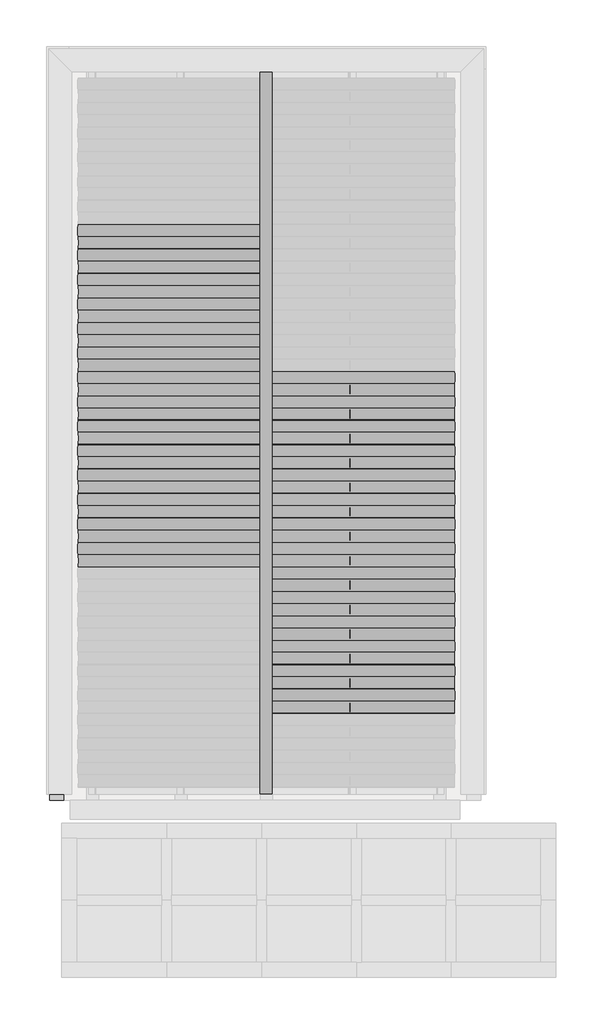
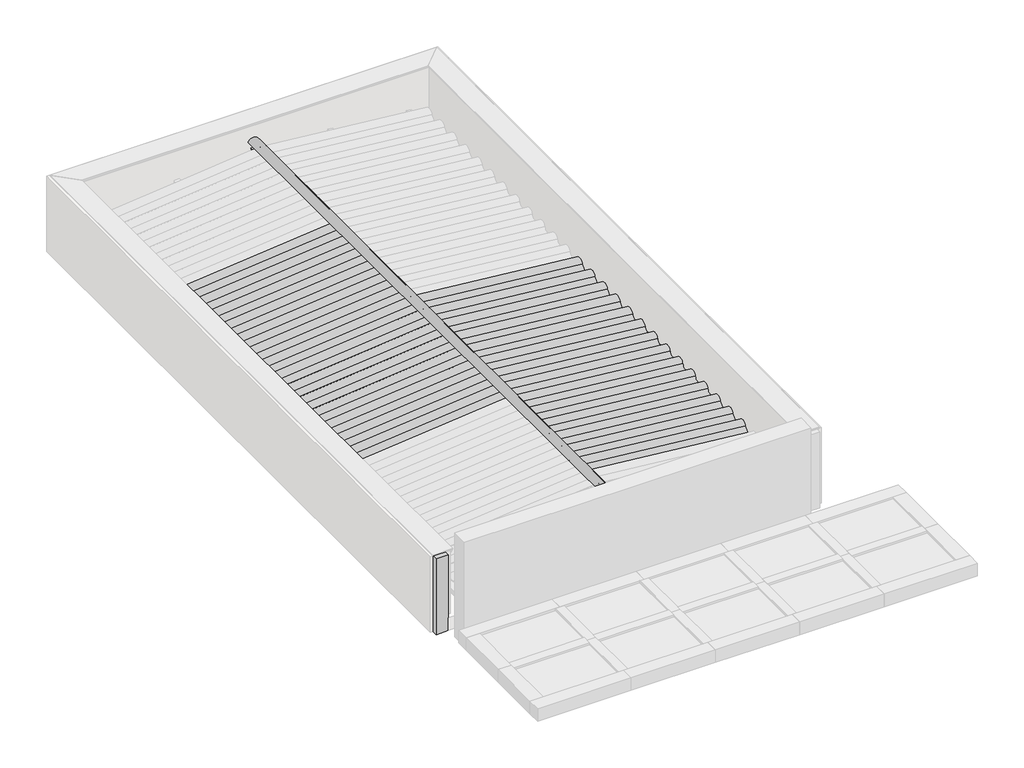
# One storey, part 2 of 3: 37 beams, 7 columns.
"""IFC4 building model written with IfcOpenShell, lengths in millimetres."""

import ifcopenshell
import ifcopenshell.guid

model = None  # the IFC model being written
_history = None  # IfcOwnerHistory: only IFC2X3 demands one
_inside = {}  # id of a spatial element -> (the spatial element, [elements in it])
_under = {}  # id of a project, library or spatial element -> (it, [spatial elements below it])
_declared = {}  # id of a project -> (the project, [libraries it declares])
_typed = {}  # id of a type object -> (the type object, [elements of that type])
_made_of = {}  # id of a material, layer set ... -> (it, [elements and type objects made of it])


def new_model(schema):
    """Start an empty IFC model of exactly this schema.

    Asked for "IFC4X3", IfcOpenShell would pick the latest addendum, in which some entities
    have other attributes; the version numbers below select the first issue.
    IFC2X3 requires an IfcOwnerHistory on every rooted entity: one is made here for all.
    """
    global model, _history
    if schema == "IFC4X3":
        model = ifcopenshell.file(schema_version=(4, 3, 0, 0))
    else:
        model = ifcopenshell.file(schema=schema)
    _inside.clear()
    _under.clear()
    _declared.clear()
    _typed.clear()
    _made_of.clear()
    _history = None
    if model.schema == "IFC2X3":
        org = make("IfcOrganization", Name="unknown")
        user = make(
            "IfcPersonAndOrganization",
            ThePerson=make("IfcPerson", FamilyName="unknown"),
            TheOrganization=org,
        )
        app = make(
            "IfcApplication",
            ApplicationDeveloper=org,
            Version="unknown",
            ApplicationFullName="unknown",
            ApplicationIdentifier="unknown",
        )
        _history = make(
            "IfcOwnerHistory",
            OwningUser=user,
            OwningApplication=app,
            ChangeAction="ADDED",
            CreationDate=0,
        )
    return model


def make(cls, **values):
    """One entity of the class cls with the attributes given. An attribute that is None is left unset."""
    return model.create_entity(
        cls, **{name: value for name, value in values.items() if value is not None}
    )


def rooted(cls, **values):
    """An entity with a GlobalId (a new one), such as an element, a storey or a relation."""
    return make(cls, GlobalId=ifcopenshell.guid.new(), OwnerHistory=_history, **values)


def si_unit(unit_type, name, prefix=None):
    """IfcSIUnit, for example si_unit("LENGTHUNIT", "METRE", prefix="MILLI")."""
    return make("IfcSIUnit", UnitType=unit_type, Prefix=prefix, Name=name)


def assignment(units):
    """IfcUnitAssignment: the units of a project."""
    return None if units is None else make("IfcUnitAssignment", Units=units)


def point(xyz):
    """IfcCartesianPoint."""
    return None if xyz is None else make("IfcCartesianPoint", Coordinates=xyz)


def direction(xyz):
    """IfcDirection."""
    return None if xyz is None else make("IfcDirection", DirectionRatios=xyz)


def frame(location, z_axis=None, x_axis=None):
    """IfcAxis2Placement3D, a coordinate frame: its origin and axes. An axis left out is left unset."""
    return make(
        "IfcAxis2Placement3D",
        Location=point(location),
        Axis=direction(z_axis),
        RefDirection=direction(x_axis),
    )


def frame_2d(location, x_axis=None):
    """IfcAxis2Placement2D, a coordinate frame in the plane: its origin and x axis."""
    return make(
        "IfcAxis2Placement2D", Location=point(location), RefDirection=direction(x_axis)
    )


def origin():
    """The frame at (0, 0, 0) with its axes left unset."""
    return frame((0.0, 0.0, 0.0))


def place(relative_to, where):
    """IfcLocalPlacement: puts the frame where relative to a parent placement (None: the world)."""
    return make(
        "IfcLocalPlacement", PlacementRelTo=relative_to, RelativePlacement=where
    )


def context(
    kind, dimensions, precision=None, world=None, true_north=None, identifier=None
):
    """IfcGeometricRepresentationContext, for example the 3D "Model" context."""
    return make(
        "IfcGeometricRepresentationContext",
        ContextIdentifier=identifier,
        ContextType=kind,
        CoordinateSpaceDimension=dimensions,
        Precision=precision,
        WorldCoordinateSystem=world,
        TrueNorth=true_north,
    )


def project(units=None, contexts=None):
    """IfcProject with its units and contexts."""
    return rooted(
        "IfcProject",
        Name="project",
        RepresentationContexts=contexts,
        UnitsInContext=assignment(units),
    )


def spatial(cls, under=None, at=None, **own):
    """A site, building, storey or space (cls), placed at a placement, below another one or the project."""
    s = rooted(cls, ObjectPlacement=at, **own)
    if under is not None:
        _under.setdefault(under.id(), (under, []))[1].append(s)
    return s


def polyline(points):
    """IfcPolyline through the points."""
    return make("IfcPolyline", Points=[point(p) for p in points])


def circle_curve(where, radius):
    """IfcCircle in the frame where."""
    return make("IfcCircle", Position=where, Radius=radius)


def trimmed(basis, trim1, trim2, sense, master):
    """IfcTrimmedCurve: the piece of a basis curve between two trims."""
    return make(
        "IfcTrimmedCurve",
        BasisCurve=basis,
        Trim1=trim1,
        Trim2=trim2,
        SenseAgreement=sense,
        MasterRepresentation=master,
    )


def segment(curve, same_sense, transition):
    """IfcCompositeCurveSegment."""
    return make(
        "IfcCompositeCurveSegment",
        Transition=transition,
        SameSense=same_sense,
        ParentCurve=curve,
    )


def composite_curve(segments, self_intersect=None):
    """IfcCompositeCurve: segments joined end to end."""
    return make("IfcCompositeCurve", Segments=segments, SelfIntersect=self_intersect)


def outline(outer, holes=None, kind="AREA"):
    """IfcArbitraryClosedProfileDef: a profile drawn as a closed curve; with holes, ...WithVoids."""
    if holes is None:
        return make("IfcArbitraryClosedProfileDef", ProfileType=kind, OuterCurve=outer)
    return make(
        "IfcArbitraryProfileDefWithVoids",
        ProfileType=kind,
        OuterCurve=outer,
        InnerCurves=holes,
    )


def extrude(swept, where, along, depth):
    """IfcExtrudedAreaSolid: the profile swept, set in the frame where, extruded along a direction by depth."""
    return make(
        "IfcExtrudedAreaSolid",
        SweptArea=swept,
        Position=where,
        ExtrudedDirection=direction(along),
        Depth=depth,
    )


def faces_of(points, faces, orient=None, outer=None):
    """IfcFace entities. A face is a list of loops; a loop is a list of indices into points, from 0.

    orient and outer hold one flag for each loop. By default every Orientation is true, the
    first loop of a face is its IfcFaceOuterBound and the others are IfcFaceBound.
    """
    made = []
    for i, loops in enumerate(faces):
        bounds = []
        for j, loop in enumerate(loops):
            is_outer = j == 0 if outer is None else outer[i][j]
            bounds.append(
                make(
                    "IfcFaceOuterBound" if is_outer else "IfcFaceBound",
                    Bound=make("IfcPolyLoop", Polygon=[points[k] for k in loop]),
                    Orientation=True if orient is None else orient[i][j],
                )
            )
        made.append(make("IfcFace", Bounds=bounds))
    return made


def faceted_brep(points, faces, orient=None, outer=None, voids=None):
    """IfcFacetedBrep: a solid bounded by flat faces; with voids (closed shells), ...WithVoids."""
    shared = [point(p) for p in points]
    hull = make("IfcClosedShell", CfsFaces=faces_of(shared, faces, orient, outer))
    if voids is None:
        return make("IfcFacetedBrep", Outer=hull)
    return make(
        "IfcFacetedBrepWithVoids",
        Outer=hull,
        Voids=[
            make(cls, CfsFaces=faces_of(shared, fs, o, b)) for cls, fs, o, b in voids
        ],
    )


def shape(context_of_items, identifier, shape_type, items):
    """IfcShapeRepresentation: the items that make up one representation, for example the "Body"."""
    return make(
        "IfcShapeRepresentation",
        ContextOfItems=context_of_items,
        RepresentationIdentifier=identifier,
        RepresentationType=shape_type,
        Items=items,
    )


def source(mapping_origin, context_of_items, identifier, shape_type, items):
    """IfcRepresentationMap: a shape defined once, which mapped items show again and again."""
    return make(
        "IfcRepresentationMap",
        MappingOrigin=mapping_origin,
        MappedRepresentation=shape(context_of_items, identifier, shape_type, items),
    )


def transform(
    local_origin,
    x_axis=None,
    y_axis=None,
    z_axis=None,
    scale=None,
    scale2=None,
    scale3=None,
    uniform=True,
):
    """IfcCartesianTransformationOperator3D, or its non-uniform kind. x_axis, y_axis, z_axis: its Axis1, 2, 3."""
    if uniform:
        return make(
            "IfcCartesianTransformationOperator3D",
            Axis1=direction(x_axis),
            Axis2=direction(y_axis),
            LocalOrigin=point(local_origin),
            Scale=scale,
            Axis3=direction(z_axis),
        )
    return make(
        "IfcCartesianTransformationOperator3DnonUniform",
        Axis1=direction(x_axis),
        Axis2=direction(y_axis),
        LocalOrigin=point(local_origin),
        Scale=scale,
        Axis3=direction(z_axis),
        Scale2=scale2,
        Scale3=scale3,
    )


def mapped(mapping_source, mapping_target):
    """IfcMappedItem: shows the shape of a source again, moved by a transform."""
    return make(
        "IfcMappedItem", MappingSource=mapping_source, MappingTarget=mapping_target
    )


def made_of(thing, what):
    """Note that an element or type object is made of a material, layer set ...; save() writes the relation."""
    if what is not None:
        _made_of.setdefault(what.id(), (what, []))[1].append(thing)
    return thing


def element(
    cls,
    number,
    at=None,
    inside=None,
    cuts=None,
    type_object=None,
    material=None,
    context=None,
    identifier="Body",
    shape_type=None,
    held_by="IfcProductDefinitionShape",
    body=None,
    shapes=None,
    **own,
):
    """One element of the class cls, such as IfcWall. Its Tag is "e" and its number.

    at: its placement. inside: the storey or other place that contains it. cuts: it is an
    opening in that element (IfcRelVoidsElement). A single representation is given by context,
    identifier, shape_type and body (its items); several are given by shapes. held_by: the class
    of the entity that holds the representations. save() writes the other relations.
    """
    e = rooted(cls, Tag="e%d" % number, ObjectPlacement=at, **own)
    if body is not None:
        shapes = [shape(context, identifier, shape_type, body)]
    if shapes is not None:
        e.Representation = make(held_by, Representations=shapes)
    if inside is not None:
        _inside.setdefault(inside.id(), (inside, []))[1].append(e)
    if cuts is not None:
        rooted(
            "IfcRelVoidsElement", RelatingBuildingElement=cuts, RelatedOpeningElement=e
        )
    if type_object is not None:
        _typed.setdefault(type_object.id(), (type_object, []))[1].append(e)
    return made_of(e, material)


def aggregate(whole, parts):
    """IfcRelAggregates: a whole, such as a stair, and the parts it consists of."""
    return rooted("IfcRelAggregates", RelatingObject=whole, RelatedObjects=parts)


def save(model, path):
    """Write the relations noted so far, then the file.

    IfcRelAggregates (storeys below a building ...), IfcRelContainedInSpatialStructure (elements
    in a storey), IfcRelDefinesByType, IfcRelAssociatesMaterial and IfcRelDeclares: one each for
    every whole, place, type object, material and project.
    """
    for whole, parts in _under.values():
        aggregate(whole, parts)
    for where, things in _inside.values():
        rooted(
            "IfcRelContainedInSpatialStructure",
            RelatedElements=things,
            RelatingStructure=where,
        )
    for kind, things in _typed.values():
        rooted("IfcRelDefinesByType", RelatedObjects=things, RelatingType=kind)
    for what, things in _made_of.values():
        rooted("IfcRelAssociatesMaterial", RelatedObjects=things, RelatingMaterial=what)
    for by, libraries in _declared.values():
        rooted("IfcRelDeclares", RelatingContext=by, RelatedDefinitions=libraries)
    model.write(path)


def cumeeira_telha_ondulada_fibrocimento_28917381(model_context):
    return source(origin(), model_context, "Body", "SweptSolid", [
        extrude(outline(composite_curve([segment(polyline([(58.3970135, 42.4437972), (53.9055884, 40.2467307)]), True, "CONTINUOUS"), segment(trimmed(circle_curve(frame_2d((-1.6029865, 13.0936483)), 61.7939461), [point((53.9055884, 40.2467307))], [point((-57.1115615, 40.2467307))], True, "CARTESIAN"), True, "CONTINUOUS"), segment(polyline([(-57.1115615, 40.2467307), (-61.6029865, 42.4437972)]), True, "CONTINUOUS"), segment(trimmed(circle_curve(frame_2d((-1.6029865, 13.0936483)), 66.7939461), [point((-61.6029865, 42.4437972))], [point((58.3970135, 42.4437972))], False, "CARTESIAN"), True, "CONTINUOUS")], self_intersect=False)), frame((-3626.5, 0.0, 0.0), z_axis=(1.0, 0.0, 0.0), x_axis=(0.0, 1.0, 0.0)), (0.0, 0.0, 1.0), 7253.0),
    ])


def viga_cumeeira_6x16cm_d80f05ee(model_context):
    return source(origin(), model_context, "Body", "SweptSolid", [
        extrude(outline(polyline([(3626.5, 30.0), (3626.5, -30.0), (-3626.5, -30.0), (-3626.5, 30.0), (3626.5, 30.0)])), frame((0.0, 0.0, -80.0), z_axis=(0.0, 0.0, 1.0), x_axis=(1.0, 0.0, 0.0)), (0.0, 0.0, 1.0), 160.0),
    ])


def column_1cffec27(model_context):
    return source(origin(), model_context, "Body", "SweptSolid", [
        extrude(outline(polyline([(30.0, 80.0), (30.0, -80.0), (-30.0, -80.0), (-30.0, 80.0), (30.0, 80.0)])), frame((0.0, 0.0, 3110.0), z_axis=(0.0, 0.0, 1.0), x_axis=(1.0, 0.0, 0.0)), (0.0, 0.0, 1.0), 238.0),
    ])


def column_35730ad5(model_context):
    return source(origin(), model_context, "Body", "SweptSolid", [
        extrude(outline(polyline([(30.0, 80.0), (30.0, -80.0), (-30.0, -80.0), (-30.0, 80.0), (30.0, 80.0)])), frame((0.0, 0.0, 3110.0), z_axis=(0.0, 0.0, 1.0), x_axis=(1.0, 0.0, 0.0)), (0.0, 0.0, 1.0), 197.9),
    ])


def column_00c463e4(model_context):
    return source(origin(), model_context, "Body", "SweptSolid", [
        extrude(outline(polyline([(30.0, 80.0), (30.0, -80.0), (-30.0, -80.0), (-30.0, 80.0), (30.0, 80.0)])), frame((0.0, 0.0, 3110.0), z_axis=(0.0, 0.0, 1.0), x_axis=(1.0, 0.0, 0.0)), (0.0, 0.0, 1.0), 109.8),
    ])


model = new_model("IFC4")

# Units and contexts
model_context = context("Model", 3, world=origin())
ifc_project = project(units=[si_unit("LENGTHUNIT", "METRE", prefix="MILLI")], contexts=[model_context])

# Site, building, storey
site = spatial("IfcSite", under=ifc_project)
building = spatial("IfcBuilding", under=site)
storey = spatial("IfcBuildingStorey", under=building, Name="COB. GARAGEM", Elevation=3050.0)

# Beams
placement = place(None, origin())
element("IfcBeam", 1, ObjectType="Madeira de lei : Berço 6x12cm", at=placement, inside=storey, context=model_context, shape_type="SweptSolid", body=[
    extrude(outline(polyline([(-9620.281307, 4423.9300153), (-9500.281307, 4423.9300153), (-9500.281307, 2423.9300153), (-9620.281307, 2423.9300153), (-9620.281307, 4423.9300153)])), frame((0.0, 0.0, 3050.0), z_axis=(0.0, 0.0, 1.0), x_axis=(1.0, 0.0, 0.0)), (0.0, 0.0, 1.0), 60.0),
])
element("IfcBeam", 2, ObjectType="Madeira de lei : Berço 6x12cm", at=placement, inside=storey, context=model_context, shape_type="SweptSolid", body=[
    extrude(outline(polyline([(-9620.281307, 2423.9300153), (-9500.281307, 2423.9300153), (-9500.281307, 423.9300153), (-9620.281307, 423.9300153), (-9620.281307, 2423.9300153)])), frame((0.0, 0.0, 3050.0), z_axis=(0.0, 0.0, 1.0), x_axis=(1.0, 0.0, 0.0)), (0.0, 0.0, 1.0), 60.0),
])
element("IfcBeam", 3, ObjectType="Madeira de lei : Berço 6x12cm", at=placement, inside=storey, context=model_context, shape_type="SweptSolid", body=[
    extrude(outline(polyline([(-8767.0824227, 4423.9300153), (-8647.0824227, 4423.9300153), (-8647.0824227, 2423.9300153), (-8767.0824227, 2423.9300153), (-8767.0824227, 4423.9300153)])), frame((0.0, 0.0, 3050.0), z_axis=(0.0, 0.0, 1.0), x_axis=(1.0, 0.0, 0.0)), (0.0, 0.0, 1.0), 60.0),
])
element("IfcBeam", 4, ObjectType="Madeira de lei : Berço 6x12cm", at=placement, inside=storey, context=model_context, shape_type="SweptSolid", body=[
    extrude(outline(polyline([(-10473.4801913, 4423.9300153), (-10353.4801913, 4423.9300153), (-10353.4801913, 2423.9300153), (-10473.4801913, 2423.9300153), (-10473.4801913, 4423.9300153)])), frame((0.0, 0.0, 3050.0), z_axis=(0.0, 0.0, 1.0), x_axis=(1.0, 0.0, 0.0)), (0.0, 0.0, 1.0), 60.0),
])
element("IfcBeam", 5, ObjectType="Madeira de lei : Berço 6x12cm", at=placement, inside=storey, context=model_context, shape_type="SweptSolid", body=[
    extrude(outline(polyline([(-11356.5301913, 4423.9300153), (-11236.5301913, 4423.9300153), (-11236.5301913, 2423.9300153), (-11356.5301913, 2423.9300153), (-11356.5301913, 4423.9300153)])), frame((0.0, 0.0, 3050.0), z_axis=(0.0, 0.0, 1.0), x_axis=(1.0, 0.0, 0.0)), (0.0, 0.0, 1.0), 60.0),
])
element("IfcBeam", 6, ObjectType="Madeira de lei : Berço 6x12cm", at=placement, inside=storey, context=model_context, shape_type="SweptSolid", body=[
    extrude(outline(polyline([(-11356.5301913, 6423.9300153), (-11236.5301913, 6423.9300153), (-11236.5301913, 4423.9300153), (-11356.5301913, 4423.9300153), (-11356.5301913, 6423.9300153)])), frame((0.0, 0.0, 3050.0), z_axis=(0.0, 0.0, 1.0), x_axis=(1.0, 0.0, 0.0)), (0.0, 0.0, 1.0), 60.0),
])
cumeeira_telha_ondulada_fibrocimento_shape = cumeeira_telha_ondulada_fibrocimento_28917381(model_context)
element("IfcBeam", 7, ObjectType="Cumeeira Telha Ondulada : Fibrocimento", at=placement, inside=storey, context=model_context, shape_type="MappedRepresentation", body=[
    mapped(cumeeira_telha_ondulada_fibrocimento_shape, transform((-9560.281307, 3455.9300153, 3545.9751229), x_axis=(0.0, -1.0, 0.0), y_axis=(1.0, 0.0, 0.0), z_axis=(0.0, 0.0, 1.0))),
])
element("IfcBeam", 8, ObjectType="TQS - Viga retangular : 14.0 x 90.0", at=placement, inside=storey, context=model_context, shape_type="Brep", body=[
    faceted_brep([(-11590.281307, 7084.4300153, 3800.0), (-11730.281307, 7084.4300153, 3800.0), (-11730.281307, -234.5699847, 3800.0), (-11590.281307, -234.5699847, 3800.0), (-11590.281307, 7084.4300153, 2900.0), (-11590.281307, 7084.4300153, 3050.0), (-11590.281307, -234.5699847, 3050.0), (-11590.281307, -234.5699847, 2900.0), (-11730.281307, 7084.4300153, 2900.0), (-11730.281307, -234.5699847, 2900.0)], [[[0, 1, 2, 3]], [[4, 5, 0, 3, 6, 7]], [[8, 4, 7, 9]], [[1, 8, 9, 2]], [[2, 9, 7, 6, 3]], [[1, 0, 5, 4, 8]]]),
])
element("IfcBeam", 9, ObjectType="Telha Ondulada : Fibrocimento", at=placement, inside=storey, context=model_context, shape_type="SweptSolid", body=[
    extrude(outline(composite_curve([segment(trimmed(circle_curve(frame_2d((-58.7002979, -53.2060538)), 66.7939461), [point((-29.350149, 6.7939462))], [point((-29.350149, -113.2060538))], False, "CARTESIAN"), True, "CONTINUOUS"), segment(polyline([(-29.350149, -113.2060538), (-31.5472155, -108.7146288)]), True, "CONTINUOUS"), segment(trimmed(circle_curve(frame_2d((-58.7002979, -53.2060538)), 61.7939461), [point((-31.5472155, -108.7146288))], [point((-31.5472155, 2.3025211))], True, "CARTESIAN"), True, "CONTINUOUS"), segment(trimmed(circle_curve(frame_2d((0.0, 66.7939462)), 71.7939461), [point((-31.5472155, 2.3025211))], [point((-31.5472155, 131.2853712))], False, "CARTESIAN"), True, "CONTINUOUS"), segment(polyline([(-31.5472155, 131.2853712), (-29.350149, 126.7939462)]), True, "CONTINUOUS"), segment(trimmed(circle_curve(frame_2d((0.0, 66.7939462)), 66.7939461), [point((-29.350149, 126.7939462))], [point((-29.350149, 6.7939462))], True, "CARTESIAN"), True, "CONTINUOUS")], self_intersect=False)), frame((-11446.918865, 2229.326948, 3394.3067746), z_axis=(0.9950371902099892, 0.0, 0.09950371902099919), x_axis=(-0.09950371902099919, 0.0, 0.9950371902099892)), (0.0, 0.0, 1.0), 1886.8678854),
])
element("IfcBeam", 10, ObjectType="Telha Ondulada : Fibrocimento", at=placement, inside=storey, context=model_context, shape_type="SweptSolid", body=[
    extrude(outline(composite_curve([segment(trimmed(circle_curve(frame_2d((-58.7002979, -53.2060538)), 66.7939461), [point((-29.350149, 6.7939462))], [point((-29.350149, -113.2060538))], False, "CARTESIAN"), True, "CONTINUOUS"), segment(polyline([(-29.350149, -113.2060538), (-31.5472155, -108.7146288)]), True, "CONTINUOUS"), segment(trimmed(circle_curve(frame_2d((-58.7002979, -53.2060538)), 61.7939461), [point((-31.5472155, -108.7146288))], [point((-31.5472155, 2.3025211))], True, "CARTESIAN"), True, "CONTINUOUS"), segment(trimmed(circle_curve(frame_2d((0.0, 66.7939462)), 71.7939461), [point((-31.5472155, 2.3025211))], [point((-31.5472155, 131.2853712))], False, "CARTESIAN"), True, "CONTINUOUS"), segment(polyline([(-31.5472155, 131.2853712), (-29.350149, 126.7939462)]), True, "CONTINUOUS"), segment(trimmed(circle_curve(frame_2d((0.0, 66.7939462)), 66.7939461), [point((-29.350149, 126.7939462))], [point((-29.350149, 6.7939462))], True, "CARTESIAN"), True, "CONTINUOUS")], self_intersect=False)), frame((-11446.918865, 2473.826948, 3394.3067746), z_axis=(0.9950371902099892, 0.0, 0.09950371902099932), x_axis=(-0.09950371902099932, 0.0, 0.9950371902099892)), (0.0, 0.0, 1.0), 1886.8678854),
])
element("IfcBeam", 11, ObjectType="Telha Ondulada : Fibrocimento", at=placement, inside=storey, context=model_context, shape_type="SweptSolid", body=[
    extrude(outline(composite_curve([segment(trimmed(circle_curve(frame_2d((-58.7002979, -53.2060538)), 66.7939461), [point((-29.350149, 6.7939462))], [point((-29.350149, -113.2060538))], False, "CARTESIAN"), True, "CONTINUOUS"), segment(polyline([(-29.350149, -113.2060538), (-31.5472155, -108.7146288)]), True, "CONTINUOUS"), segment(trimmed(circle_curve(frame_2d((-58.7002979, -53.2060538)), 61.7939461), [point((-31.5472155, -108.7146288))], [point((-31.5472155, 2.3025211))], True, "CARTESIAN"), True, "CONTINUOUS"), segment(trimmed(circle_curve(frame_2d((0.0, 66.7939462)), 71.7939461), [point((-31.5472155, 2.3025211))], [point((-31.5472155, 131.2853712))], False, "CARTESIAN"), True, "CONTINUOUS"), segment(polyline([(-31.5472155, 131.2853712), (-29.350149, 126.7939462)]), True, "CONTINUOUS"), segment(trimmed(circle_curve(frame_2d((0.0, 66.7939462)), 66.7939461), [point((-29.350149, 126.7939462))], [point((-29.350149, 6.7939462))], True, "CARTESIAN"), True, "CONTINUOUS")], self_intersect=False)), frame((-11446.918865, 2718.326948, 3394.3067746), z_axis=(0.9950371902099892, 0.0, 0.09950371902099937), x_axis=(-0.09950371902099937, 0.0, 0.9950371902099892)), (0.0, 0.0, 1.0), 1886.8678854),
])
element("IfcBeam", 12, ObjectType="Telha Ondulada : Fibrocimento", at=placement, inside=storey, context=model_context, shape_type="SweptSolid", body=[
    extrude(outline(composite_curve([segment(trimmed(circle_curve(frame_2d((-58.7002979, -53.2060538)), 66.7939461), [point((-29.350149, 6.7939462))], [point((-29.350149, -113.2060538))], False, "CARTESIAN"), True, "CONTINUOUS"), segment(polyline([(-29.350149, -113.2060538), (-31.5472155, -108.7146288)]), True, "CONTINUOUS"), segment(trimmed(circle_curve(frame_2d((-58.7002979, -53.2060538)), 61.7939461), [point((-31.5472155, -108.7146288))], [point((-31.5472155, 2.3025211))], True, "CARTESIAN"), True, "CONTINUOUS"), segment(trimmed(circle_curve(frame_2d((0.0, 66.7939462)), 71.7939461), [point((-31.5472155, 2.3025211))], [point((-31.5472155, 131.2853712))], False, "CARTESIAN"), True, "CONTINUOUS"), segment(polyline([(-31.5472155, 131.2853712), (-29.350149, 126.7939462)]), True, "CONTINUOUS"), segment(trimmed(circle_curve(frame_2d((0.0, 66.7939462)), 66.7939461), [point((-29.350149, 126.7939462))], [point((-29.350149, 6.7939462))], True, "CARTESIAN"), True, "CONTINUOUS")], self_intersect=False)), frame((-11446.918865, 2962.826948, 3394.3067746), z_axis=(0.9950371902099892, 0.0, 0.09950371902099943), x_axis=(-0.09950371902099943, 0.0, 0.9950371902099892)), (0.0, 0.0, 1.0), 1886.8678854),
])
element("IfcBeam", 13, ObjectType="Telha Ondulada : Fibrocimento", at=placement, inside=storey, context=model_context, shape_type="SweptSolid", body=[
    extrude(outline(composite_curve([segment(trimmed(circle_curve(frame_2d((-58.7002979, -53.2060538)), 66.7939461), [point((-29.350149, 6.7939462))], [point((-29.350149, -113.2060538))], False, "CARTESIAN"), True, "CONTINUOUS"), segment(polyline([(-29.350149, -113.2060538), (-31.5472155, -108.7146288)]), True, "CONTINUOUS"), segment(trimmed(circle_curve(frame_2d((-58.7002979, -53.2060538)), 61.7939461), [point((-31.5472155, -108.7146288))], [point((-31.5472155, 2.3025211))], True, "CARTESIAN"), True, "CONTINUOUS"), segment(trimmed(circle_curve(frame_2d((0.0, 66.7939462)), 71.7939461), [point((-31.5472155, 2.3025211))], [point((-31.5472155, 131.2853712))], False, "CARTESIAN"), True, "CONTINUOUS"), segment(polyline([(-31.5472155, 131.2853712), (-29.350149, 126.7939462)]), True, "CONTINUOUS"), segment(trimmed(circle_curve(frame_2d((0.0, 66.7939462)), 66.7939461), [point((-29.350149, 126.7939462))], [point((-29.350149, 6.7939462))], True, "CARTESIAN"), True, "CONTINUOUS")], self_intersect=False)), frame((-11446.918865, 3207.326948, 3394.3067746), z_axis=(0.9950371902099892, 0.0, 0.09950371902099954), x_axis=(-0.09950371902099954, 0.0, 0.9950371902099892)), (0.0, 0.0, 1.0), 1886.8678854),
])
element("IfcBeam", 14, ObjectType="Telha Ondulada : Fibrocimento", at=placement, inside=storey, context=model_context, shape_type="SweptSolid", body=[
    extrude(outline(composite_curve([segment(trimmed(circle_curve(frame_2d((-58.7002979, -53.2060538)), 66.7939461), [point((-29.350149, 6.7939462))], [point((-29.350149, -113.2060538))], False, "CARTESIAN"), True, "CONTINUOUS"), segment(polyline([(-29.350149, -113.2060538), (-31.5472155, -108.7146288)]), True, "CONTINUOUS"), segment(trimmed(circle_curve(frame_2d((-58.7002979, -53.2060538)), 61.7939461), [point((-31.5472155, -108.7146288))], [point((-31.5472155, 2.3025211))], True, "CARTESIAN"), True, "CONTINUOUS"), segment(trimmed(circle_curve(frame_2d((0.0, 66.7939462)), 71.7939461), [point((-31.5472155, 2.3025211))], [point((-31.5472155, 131.2853712))], False, "CARTESIAN"), True, "CONTINUOUS"), segment(polyline([(-31.5472155, 131.2853712), (-29.350149, 126.7939462)]), True, "CONTINUOUS"), segment(trimmed(circle_curve(frame_2d((0.0, 66.7939462)), 66.7939461), [point((-29.350149, 126.7939462))], [point((-29.350149, 6.7939462))], True, "CARTESIAN"), True, "CONTINUOUS")], self_intersect=False)), frame((-11446.918865, 3451.826948, 3394.3067746), z_axis=(0.9950371902099892, 0.0, 0.09950371902099937), x_axis=(-0.09950371902099937, 0.0, 0.9950371902099892)), (0.0, 0.0, 1.0), 1886.8678854),
])
element("IfcBeam", 15, ObjectType="Telha Ondulada : Fibrocimento", at=placement, inside=storey, context=model_context, shape_type="SweptSolid", body=[
    extrude(outline(composite_curve([segment(trimmed(circle_curve(frame_2d((-58.7002979, -53.2060538)), 66.7939461), [point((-29.350149, 6.7939462))], [point((-29.350149, -113.2060538))], False, "CARTESIAN"), True, "CONTINUOUS"), segment(polyline([(-29.350149, -113.2060538), (-31.5472155, -108.7146288)]), True, "CONTINUOUS"), segment(trimmed(circle_curve(frame_2d((-58.7002979, -53.2060538)), 61.7939461), [point((-31.5472155, -108.7146288))], [point((-31.5472155, 2.3025211))], True, "CARTESIAN"), True, "CONTINUOUS"), segment(trimmed(circle_curve(frame_2d((0.0, 66.7939462)), 71.7939461), [point((-31.5472155, 2.3025211))], [point((-31.5472155, 131.2853712))], False, "CARTESIAN"), True, "CONTINUOUS"), segment(polyline([(-31.5472155, 131.2853712), (-29.350149, 126.7939462)]), True, "CONTINUOUS"), segment(trimmed(circle_curve(frame_2d((0.0, 66.7939462)), 66.7939461), [point((-29.350149, 126.7939462))], [point((-29.350149, 6.7939462))], True, "CARTESIAN"), True, "CONTINUOUS")], self_intersect=False)), frame((-11446.918865, 3696.326948, 3394.3067746), z_axis=(0.9950371902099892, 0.0, 0.09950371902099914), x_axis=(-0.09950371902099914, 0.0, 0.9950371902099892)), (0.0, 0.0, 1.0), 1886.8678854),
])
element("IfcBeam", 16, ObjectType="Telha Ondulada : Fibrocimento", at=placement, inside=storey, context=model_context, shape_type="SweptSolid", body=[
    extrude(outline(composite_curve([segment(trimmed(circle_curve(frame_2d((-58.7002979, -53.2060538)), 66.7939461), [point((-29.350149, 6.7939462))], [point((-29.350149, -113.2060538))], False, "CARTESIAN"), True, "CONTINUOUS"), segment(polyline([(-29.350149, -113.2060538), (-31.5472155, -108.7146288)]), True, "CONTINUOUS"), segment(trimmed(circle_curve(frame_2d((-58.7002979, -53.2060538)), 61.7939461), [point((-31.5472155, -108.7146288))], [point((-31.5472155, 2.3025211))], True, "CARTESIAN"), True, "CONTINUOUS"), segment(trimmed(circle_curve(frame_2d((0.0, 66.7939462)), 71.7939461), [point((-31.5472155, 2.3025211))], [point((-31.5472155, 131.2853712))], False, "CARTESIAN"), True, "CONTINUOUS"), segment(polyline([(-31.5472155, 131.2853712), (-29.350149, 126.7939462)]), True, "CONTINUOUS"), segment(trimmed(circle_curve(frame_2d((0.0, 66.7939462)), 66.7939461), [point((-29.350149, 126.7939462))], [point((-29.350149, 6.7939462))], True, "CARTESIAN"), True, "CONTINUOUS")], self_intersect=False)), frame((-11446.918865, 3940.826948, 3394.3067746), z_axis=(0.9950371902099892, 0.0, 0.09950371902099948), x_axis=(-0.09950371902099948, 0.0, 0.9950371902099892)), (0.0, 0.0, 1.0), 1886.8678854),
])
element("IfcBeam", 17, ObjectType="Telha Ondulada : Fibrocimento", at=placement, inside=storey, context=model_context, shape_type="SweptSolid", body=[
    extrude(outline(composite_curve([segment(trimmed(circle_curve(frame_2d((-58.7002979, -53.2060538)), 66.7939461), [point((-29.350149, 6.7939462))], [point((-29.350149, -113.2060538))], False, "CARTESIAN"), True, "CONTINUOUS"), segment(polyline([(-29.350149, -113.2060538), (-31.5472155, -108.7146288)]), True, "CONTINUOUS"), segment(trimmed(circle_curve(frame_2d((-58.7002979, -53.2060538)), 61.7939461), [point((-31.5472155, -108.7146288))], [point((-31.5472155, 2.3025211))], True, "CARTESIAN"), True, "CONTINUOUS"), segment(trimmed(circle_curve(frame_2d((0.0, 66.7939462)), 71.7939461), [point((-31.5472155, 2.3025211))], [point((-31.5472155, 131.2853712))], False, "CARTESIAN"), True, "CONTINUOUS"), segment(polyline([(-31.5472155, 131.2853712), (-29.350149, 126.7939462)]), True, "CONTINUOUS"), segment(trimmed(circle_curve(frame_2d((0.0, 66.7939462)), 66.7939461), [point((-29.350149, 126.7939462))], [point((-29.350149, 6.7939462))], True, "CARTESIAN"), True, "CONTINUOUS")], self_intersect=False)), frame((-11446.918865, 4185.326948, 3394.3067746), z_axis=(0.9950371902099892, 0.0, 0.09950371902099932), x_axis=(-0.09950371902099932, 0.0, 0.9950371902099892)), (0.0, 0.0, 1.0), 1886.8678854),
])
element("IfcBeam", 18, ObjectType="Telha Ondulada : Fibrocimento", at=placement, inside=storey, context=model_context, shape_type="SweptSolid", body=[
    extrude(outline(composite_curve([segment(trimmed(circle_curve(frame_2d((-58.7002979, -53.2060538)), 66.7939461), [point((-29.350149, 6.7939462))], [point((-29.350149, -113.2060538))], False, "CARTESIAN"), True, "CONTINUOUS"), segment(polyline([(-29.350149, -113.2060538), (-31.5472155, -108.7146288)]), True, "CONTINUOUS"), segment(trimmed(circle_curve(frame_2d((-58.7002979, -53.2060538)), 61.7939461), [point((-31.5472155, -108.7146288))], [point((-31.5472155, 2.3025211))], True, "CARTESIAN"), True, "CONTINUOUS"), segment(trimmed(circle_curve(frame_2d((0.0, 66.7939462)), 71.7939461), [point((-31.5472155, 2.3025211))], [point((-31.5472155, 131.2853712))], False, "CARTESIAN"), True, "CONTINUOUS"), segment(polyline([(-31.5472155, 131.2853712), (-29.350149, 126.7939462)]), True, "CONTINUOUS"), segment(trimmed(circle_curve(frame_2d((0.0, 66.7939462)), 66.7939461), [point((-29.350149, 126.7939462))], [point((-29.350149, 6.7939462))], True, "CARTESIAN"), True, "CONTINUOUS")], self_intersect=False)), frame((-11446.918865, 4429.826948, 3394.3067746), z_axis=(0.9950371902099892, 0.0, 0.09950371902099943), x_axis=(-0.09950371902099943, 0.0, 0.9950371902099892)), (0.0, 0.0, 1.0), 1886.8678854),
])
element("IfcBeam", 19, ObjectType="Telha Ondulada : Fibrocimento", at=placement, inside=storey, context=model_context, shape_type="SweptSolid", body=[
    extrude(outline(composite_curve([segment(trimmed(circle_curve(frame_2d((-58.7002979, -53.2060538)), 66.7939461), [point((-29.350149, 6.7939462))], [point((-29.350149, -113.2060538))], False, "CARTESIAN"), True, "CONTINUOUS"), segment(polyline([(-29.350149, -113.2060538), (-31.5472155, -108.7146288)]), True, "CONTINUOUS"), segment(trimmed(circle_curve(frame_2d((-58.7002979, -53.2060538)), 61.7939461), [point((-31.5472155, -108.7146288))], [point((-31.5472155, 2.3025211))], True, "CARTESIAN"), True, "CONTINUOUS"), segment(trimmed(circle_curve(frame_2d((0.0, 66.7939462)), 71.7939461), [point((-31.5472155, 2.3025211))], [point((-31.5472155, 131.2853712))], False, "CARTESIAN"), True, "CONTINUOUS"), segment(polyline([(-31.5472155, 131.2853712), (-29.350149, 126.7939462)]), True, "CONTINUOUS"), segment(trimmed(circle_curve(frame_2d((0.0, 66.7939462)), 66.7939461), [point((-29.350149, 126.7939462))], [point((-29.350149, 6.7939462))], True, "CARTESIAN"), True, "CONTINUOUS")], self_intersect=False)), frame((-11446.918865, 4674.326948, 3394.3067746), z_axis=(0.9950371902099892, 0.0, 0.09950371902099943), x_axis=(-0.09950371902099943, 0.0, 0.9950371902099892)), (0.0, 0.0, 1.0), 1886.8678854),
])
element("IfcBeam", 20, ObjectType="Telha Ondulada : Fibrocimento", at=placement, inside=storey, context=model_context, shape_type="SweptSolid", body=[
    extrude(outline(composite_curve([segment(trimmed(circle_curve(frame_2d((-58.7002979, -53.2060538)), 66.7939461), [point((-29.350149, 6.7939462))], [point((-29.350149, -113.2060538))], False, "CARTESIAN"), True, "CONTINUOUS"), segment(polyline([(-29.350149, -113.2060538), (-31.5472155, -108.7146288)]), True, "CONTINUOUS"), segment(trimmed(circle_curve(frame_2d((-58.7002979, -53.2060538)), 61.7939461), [point((-31.5472155, -108.7146288))], [point((-31.5472155, 2.3025211))], True, "CARTESIAN"), True, "CONTINUOUS"), segment(trimmed(circle_curve(frame_2d((0.0, 66.7939462)), 71.7939461), [point((-31.5472155, 2.3025211))], [point((-31.5472155, 131.2853712))], False, "CARTESIAN"), True, "CONTINUOUS"), segment(polyline([(-31.5472155, 131.2853712), (-29.350149, 126.7939462)]), True, "CONTINUOUS"), segment(trimmed(circle_curve(frame_2d((0.0, 66.7939462)), 66.7939461), [point((-29.350149, 126.7939462))], [point((-29.350149, 6.7939462))], True, "CARTESIAN"), True, "CONTINUOUS")], self_intersect=False)), frame((-11446.918865, 4918.826948, 3394.3067746), z_axis=(0.9950371902099892, 0.0, 0.09950371902099903), x_axis=(-0.09950371902099903, 0.0, 0.9950371902099892)), (0.0, 0.0, 1.0), 1886.8678854),
])
element("IfcBeam", 21, ObjectType="Telha Ondulada : Fibrocimento", at=placement, inside=storey, context=model_context, shape_type="SweptSolid", body=[
    extrude(outline(composite_curve([segment(trimmed(circle_curve(frame_2d((-58.7002979, -53.2060538)), 66.7939461), [point((-29.350149, 6.7939462))], [point((-29.350149, -113.2060538))], False, "CARTESIAN"), True, "CONTINUOUS"), segment(polyline([(-29.350149, -113.2060538), (-31.5472155, -108.7146288)]), True, "CONTINUOUS"), segment(trimmed(circle_curve(frame_2d((-58.7002979, -53.2060538)), 61.7939461), [point((-31.5472155, -108.7146288))], [point((-31.5472155, 2.3025211))], True, "CARTESIAN"), True, "CONTINUOUS"), segment(trimmed(circle_curve(frame_2d((0.0, 66.7939462)), 71.7939461), [point((-31.5472155, 2.3025211))], [point((-31.5472155, 131.2853712))], False, "CARTESIAN"), True, "CONTINUOUS"), segment(polyline([(-31.5472155, 131.2853712), (-29.350149, 126.7939462)]), True, "CONTINUOUS"), segment(trimmed(circle_curve(frame_2d((0.0, 66.7939462)), 66.7939461), [point((-29.350149, 126.7939462))], [point((-29.350149, 6.7939462))], True, "CARTESIAN"), True, "CONTINUOUS")], self_intersect=False)), frame((-11446.918865, 5163.326948, 3394.3067746), z_axis=(0.9950371902099892, 0.0, 0.09950371902099937), x_axis=(-0.09950371902099937, 0.0, 0.9950371902099892)), (0.0, 0.0, 1.0), 1886.8678854),
])
element("IfcBeam", 22, ObjectType="Telha Ondulada : Fibrocimento", at=placement, inside=storey, context=model_context, shape_type="SweptSolid", body=[
    extrude(outline(composite_curve([segment(trimmed(circle_curve(frame_2d((-58.7002979, -53.2060538)), 66.7939461), [point((-29.350149, 6.7939462))], [point((-29.350149, -113.2060538))], False, "CARTESIAN"), True, "CONTINUOUS"), segment(polyline([(-29.350149, -113.2060538), (-31.5472155, -108.7146288)]), True, "CONTINUOUS"), segment(trimmed(circle_curve(frame_2d((-58.7002979, -53.2060538)), 61.7939461), [point((-31.5472155, -108.7146288))], [point((-31.5472155, 2.3025211))], True, "CARTESIAN"), True, "CONTINUOUS"), segment(trimmed(circle_curve(frame_2d((0.0, 66.7939462)), 71.7939461), [point((-31.5472155, 2.3025211))], [point((-31.5472155, 131.2853712))], False, "CARTESIAN"), True, "CONTINUOUS"), segment(polyline([(-31.5472155, 131.2853712), (-29.350149, 126.7939462)]), True, "CONTINUOUS"), segment(trimmed(circle_curve(frame_2d((0.0, 66.7939462)), 66.7939461), [point((-29.350149, 126.7939462))], [point((-29.350149, 6.7939462))], True, "CARTESIAN"), True, "CONTINUOUS")], self_intersect=False)), frame((-11446.918865, 5407.826948, 3394.3067746), z_axis=(0.9950371902099892, 0.0, 0.09950371902099972), x_axis=(-0.09950371902099972, 0.0, 0.9950371902099892)), (0.0, 0.0, 1.0), 1886.8678854),
])
element("IfcBeam", 23, ObjectType="Telha Ondulada : Fibrocimento", at=placement, inside=storey, context=model_context, shape_type="SweptSolid", body=[
    extrude(outline(composite_curve([segment(trimmed(circle_curve(frame_2d((0.0, 66.7939462)), 66.7939461), [point((29.350149, 6.7939462))], [point((29.350149, 126.7939462))], True, "CARTESIAN"), True, "CONTINUOUS"), segment(polyline([(29.350149, 126.7939462), (31.5472155, 131.2853712)]), True, "CONTINUOUS"), segment(trimmed(circle_curve(frame_2d((0.0, 66.7939462)), 71.7939461), [point((31.5472155, 131.2853712))], [point((31.5472155, 2.3025211))], False, "CARTESIAN"), True, "CONTINUOUS"), segment(trimmed(circle_curve(frame_2d((58.7002979, -53.2060538)), 61.7939461), [point((31.5472155, 2.3025211))], [point((31.5472155, -108.7146288))], True, "CARTESIAN"), True, "CONTINUOUS"), segment(polyline([(31.5472155, -108.7146288), (29.350149, -113.2060538)]), True, "CONTINUOUS"), segment(trimmed(circle_curve(frame_2d((58.7002979, -53.2060538)), 66.7939461), [point((29.350149, -113.2060538))], [point((29.350149, 6.7939462))], False, "CARTESIAN"), True, "CONTINUOUS")], self_intersect=False)), frame((-7673.6437489, 762.326948, 3394.3067746), z_axis=(-0.9950371902099892, 0.0, 0.09950371902099965), x_axis=(-0.09950371902099965, 0.0, -0.9950371902099892)), (0.0, 0.0, 1.0), 1886.8678854),
])
element("IfcBeam", 24, ObjectType="Telha Ondulada : Fibrocimento", at=placement, inside=storey, context=model_context, shape_type="SweptSolid", body=[
    extrude(outline(composite_curve([segment(trimmed(circle_curve(frame_2d((0.0, 66.7939462)), 66.7939461), [point((29.350149, 6.7939462))], [point((29.350149, 126.7939462))], True, "CARTESIAN"), True, "CONTINUOUS"), segment(polyline([(29.350149, 126.7939462), (31.5472155, 131.2853712)]), True, "CONTINUOUS"), segment(trimmed(circle_curve(frame_2d((0.0, 66.7939462)), 71.7939461), [point((31.5472155, 131.2853712))], [point((31.5472155, 2.3025211))], False, "CARTESIAN"), True, "CONTINUOUS"), segment(trimmed(circle_curve(frame_2d((58.7002979, -53.2060538)), 61.7939461), [point((31.5472155, 2.3025211))], [point((31.5472155, -108.7146288))], True, "CARTESIAN"), True, "CONTINUOUS"), segment(polyline([(31.5472155, -108.7146288), (29.350149, -113.2060538)]), True, "CONTINUOUS"), segment(trimmed(circle_curve(frame_2d((58.7002979, -53.2060538)), 66.7939461), [point((29.350149, -113.2060538))], [point((29.350149, 6.7939462))], False, "CARTESIAN"), True, "CONTINUOUS")], self_intersect=False)), frame((-7673.6437489, 1006.826948, 3394.3067746), z_axis=(-0.9950371902099892, 0.0, 0.09950371902099965), x_axis=(-0.09950371902099965, 0.0, -0.9950371902099892)), (0.0, 0.0, 1.0), 1886.8678854),
])
element("IfcBeam", 25, ObjectType="Telha Ondulada : Fibrocimento", at=placement, inside=storey, context=model_context, shape_type="SweptSolid", body=[
    extrude(outline(composite_curve([segment(trimmed(circle_curve(frame_2d((0.0, 66.7939462)), 66.7939461), [point((29.350149, 6.7939462))], [point((29.350149, 126.7939462))], True, "CARTESIAN"), True, "CONTINUOUS"), segment(polyline([(29.350149, 126.7939462), (31.5472155, 131.2853712)]), True, "CONTINUOUS"), segment(trimmed(circle_curve(frame_2d((0.0, 66.7939462)), 71.7939461), [point((31.5472155, 131.2853712))], [point((31.5472155, 2.3025211))], False, "CARTESIAN"), True, "CONTINUOUS"), segment(trimmed(circle_curve(frame_2d((58.7002979, -53.2060538)), 61.7939461), [point((31.5472155, 2.3025211))], [point((31.5472155, -108.7146288))], True, "CARTESIAN"), True, "CONTINUOUS"), segment(polyline([(31.5472155, -108.7146288), (29.350149, -113.2060538)]), True, "CONTINUOUS"), segment(trimmed(circle_curve(frame_2d((58.7002979, -53.2060538)), 66.7939461), [point((29.350149, -113.2060538))], [point((29.350149, 6.7939462))], False, "CARTESIAN"), True, "CONTINUOUS")], self_intersect=False)), frame((-7673.6437489, 1251.326948, 3394.3067746), z_axis=(-0.9950371902099892, 0.0, 0.09950371902099965), x_axis=(-0.09950371902099965, 0.0, -0.9950371902099892)), (0.0, 0.0, 1.0), 1886.8678854),
])
element("IfcBeam", 26, ObjectType="Telha Ondulada : Fibrocimento", at=placement, inside=storey, context=model_context, shape_type="SweptSolid", body=[
    extrude(outline(composite_curve([segment(trimmed(circle_curve(frame_2d((0.0, 66.7939462)), 66.7939461), [point((29.350149, 6.7939462))], [point((29.350149, 126.7939462))], True, "CARTESIAN"), True, "CONTINUOUS"), segment(polyline([(29.350149, 126.7939462), (31.5472155, 131.2853712)]), True, "CONTINUOUS"), segment(trimmed(circle_curve(frame_2d((0.0, 66.7939462)), 71.7939461), [point((31.5472155, 131.2853712))], [point((31.5472155, 2.3025211))], False, "CARTESIAN"), True, "CONTINUOUS"), segment(trimmed(circle_curve(frame_2d((58.7002979, -53.2060538)), 61.7939461), [point((31.5472155, 2.3025211))], [point((31.5472155, -108.7146288))], True, "CARTESIAN"), True, "CONTINUOUS"), segment(polyline([(31.5472155, -108.7146288), (29.350149, -113.2060538)]), True, "CONTINUOUS"), segment(trimmed(circle_curve(frame_2d((58.7002979, -53.2060538)), 66.7939461), [point((29.350149, -113.2060538))], [point((29.350149, 6.7939462))], False, "CARTESIAN"), True, "CONTINUOUS")], self_intersect=False)), frame((-7673.6437489, 1495.826948, 3394.3067746), z_axis=(-0.9950371902099892, 0.0, 0.09950371902099965), x_axis=(-0.09950371902099965, 0.0, -0.9950371902099892)), (0.0, 0.0, 1.0), 1886.8678854),
])
element("IfcBeam", 27, ObjectType="Telha Ondulada : Fibrocimento", at=placement, inside=storey, context=model_context, shape_type="SweptSolid", body=[
    extrude(outline(composite_curve([segment(trimmed(circle_curve(frame_2d((0.0, 66.7939462)), 66.7939461), [point((29.350149, 6.7939462))], [point((29.350149, 126.7939462))], True, "CARTESIAN"), True, "CONTINUOUS"), segment(polyline([(29.350149, 126.7939462), (31.5472155, 131.2853712)]), True, "CONTINUOUS"), segment(trimmed(circle_curve(frame_2d((0.0, 66.7939462)), 71.7939461), [point((31.5472155, 131.2853712))], [point((31.5472155, 2.3025211))], False, "CARTESIAN"), True, "CONTINUOUS"), segment(trimmed(circle_curve(frame_2d((58.7002979, -53.2060538)), 61.7939461), [point((31.5472155, 2.3025211))], [point((31.5472155, -108.7146288))], True, "CARTESIAN"), True, "CONTINUOUS"), segment(polyline([(31.5472155, -108.7146288), (29.350149, -113.2060538)]), True, "CONTINUOUS"), segment(trimmed(circle_curve(frame_2d((58.7002979, -53.2060538)), 66.7939461), [point((29.350149, -113.2060538))], [point((29.350149, 6.7939462))], False, "CARTESIAN"), True, "CONTINUOUS")], self_intersect=False)), frame((-7673.6437489, 1740.326948, 3394.3067746), z_axis=(-0.9950371902099892, 0.0, 0.09950371902099965), x_axis=(-0.09950371902099965, 0.0, -0.9950371902099892)), (0.0, 0.0, 1.0), 1886.8678854),
])
element("IfcBeam", 28, ObjectType="Telha Ondulada : Fibrocimento", at=placement, inside=storey, context=model_context, shape_type="SweptSolid", body=[
    extrude(outline(composite_curve([segment(trimmed(circle_curve(frame_2d((0.0, 66.7939462)), 66.7939461), [point((29.350149, 6.7939462))], [point((29.350149, 126.7939462))], True, "CARTESIAN"), True, "CONTINUOUS"), segment(polyline([(29.350149, 126.7939462), (31.5472155, 131.2853712)]), True, "CONTINUOUS"), segment(trimmed(circle_curve(frame_2d((0.0, 66.7939462)), 71.7939461), [point((31.5472155, 131.2853712))], [point((31.5472155, 2.3025211))], False, "CARTESIAN"), True, "CONTINUOUS"), segment(trimmed(circle_curve(frame_2d((58.7002979, -53.2060538)), 61.7939461), [point((31.5472155, 2.3025211))], [point((31.5472155, -108.7146288))], True, "CARTESIAN"), True, "CONTINUOUS"), segment(polyline([(31.5472155, -108.7146288), (29.350149, -113.2060538)]), True, "CONTINUOUS"), segment(trimmed(circle_curve(frame_2d((58.7002979, -53.2060538)), 66.7939461), [point((29.350149, -113.2060538))], [point((29.350149, 6.7939462))], False, "CARTESIAN"), True, "CONTINUOUS")], self_intersect=False)), frame((-7673.6437489, 1984.826948, 3394.3067746), z_axis=(-0.9950371902099892, 0.0, 0.09950371902099965), x_axis=(-0.09950371902099965, 0.0, -0.9950371902099892)), (0.0, 0.0, 1.0), 1886.8678854),
])
element("IfcBeam", 29, ObjectType="Telha Ondulada : Fibrocimento", at=placement, inside=storey, context=model_context, shape_type="SweptSolid", body=[
    extrude(outline(composite_curve([segment(trimmed(circle_curve(frame_2d((0.0, 66.7939462)), 66.7939461), [point((29.350149, 6.7939462))], [point((29.350149, 126.7939462))], True, "CARTESIAN"), True, "CONTINUOUS"), segment(polyline([(29.350149, 126.7939462), (31.5472155, 131.2853712)]), True, "CONTINUOUS"), segment(trimmed(circle_curve(frame_2d((0.0, 66.7939462)), 71.7939461), [point((31.5472155, 131.2853712))], [point((31.5472155, 2.3025211))], False, "CARTESIAN"), True, "CONTINUOUS"), segment(trimmed(circle_curve(frame_2d((58.7002979, -53.2060538)), 61.7939461), [point((31.5472155, 2.3025211))], [point((31.5472155, -108.7146288))], True, "CARTESIAN"), True, "CONTINUOUS"), segment(polyline([(31.5472155, -108.7146288), (29.350149, -113.2060538)]), True, "CONTINUOUS"), segment(trimmed(circle_curve(frame_2d((58.7002979, -53.2060538)), 66.7939461), [point((29.350149, -113.2060538))], [point((29.350149, 6.7939462))], False, "CARTESIAN"), True, "CONTINUOUS")], self_intersect=False)), frame((-7673.6437489, 2229.326948, 3394.3067746), z_axis=(-0.9950371902099892, 0.0, 0.09950371902099965), x_axis=(-0.09950371902099965, 0.0, -0.9950371902099892)), (0.0, 0.0, 1.0), 1886.8678854),
])
element("IfcBeam", 30, ObjectType="Telha Ondulada : Fibrocimento", at=placement, inside=storey, context=model_context, shape_type="SweptSolid", body=[
    extrude(outline(composite_curve([segment(trimmed(circle_curve(frame_2d((0.0, 66.7939462)), 66.7939461), [point((29.350149, 6.7939462))], [point((29.350149, 126.7939462))], True, "CARTESIAN"), True, "CONTINUOUS"), segment(polyline([(29.350149, 126.7939462), (31.5472155, 131.2853712)]), True, "CONTINUOUS"), segment(trimmed(circle_curve(frame_2d((0.0, 66.7939462)), 71.7939461), [point((31.5472155, 131.2853712))], [point((31.5472155, 2.3025211))], False, "CARTESIAN"), True, "CONTINUOUS"), segment(trimmed(circle_curve(frame_2d((58.7002979, -53.2060538)), 61.7939461), [point((31.5472155, 2.3025211))], [point((31.5472155, -108.7146288))], True, "CARTESIAN"), True, "CONTINUOUS"), segment(polyline([(31.5472155, -108.7146288), (29.350149, -113.2060538)]), True, "CONTINUOUS"), segment(trimmed(circle_curve(frame_2d((58.7002979, -53.2060538)), 66.7939461), [point((29.350149, -113.2060538))], [point((29.350149, 6.7939462))], False, "CARTESIAN"), True, "CONTINUOUS")], self_intersect=False)), frame((-7673.6437489, 2473.826948, 3394.3067746), z_axis=(-0.9950371902099892, 0.0, 0.09950371902099965), x_axis=(-0.09950371902099965, 0.0, -0.9950371902099892)), (0.0, 0.0, 1.0), 1886.8678854),
])
element("IfcBeam", 31, ObjectType="Telha Ondulada : Fibrocimento", at=placement, inside=storey, context=model_context, shape_type="SweptSolid", body=[
    extrude(outline(composite_curve([segment(trimmed(circle_curve(frame_2d((0.0, 66.7939462)), 66.7939461), [point((29.350149, 6.7939462))], [point((29.350149, 126.7939462))], True, "CARTESIAN"), True, "CONTINUOUS"), segment(polyline([(29.350149, 126.7939462), (31.5472155, 131.2853712)]), True, "CONTINUOUS"), segment(trimmed(circle_curve(frame_2d((0.0, 66.7939462)), 71.7939461), [point((31.5472155, 131.2853712))], [point((31.5472155, 2.3025211))], False, "CARTESIAN"), True, "CONTINUOUS"), segment(trimmed(circle_curve(frame_2d((58.7002979, -53.2060538)), 61.7939461), [point((31.5472155, 2.3025211))], [point((31.5472155, -108.7146288))], True, "CARTESIAN"), True, "CONTINUOUS"), segment(polyline([(31.5472155, -108.7146288), (29.350149, -113.2060538)]), True, "CONTINUOUS"), segment(trimmed(circle_curve(frame_2d((58.7002979, -53.2060538)), 66.7939461), [point((29.350149, -113.2060538))], [point((29.350149, 6.7939462))], False, "CARTESIAN"), True, "CONTINUOUS")], self_intersect=False)), frame((-7673.6437489, 2718.326948, 3394.3067746), z_axis=(-0.9950371902099892, 0.0, 0.09950371902099965), x_axis=(-0.09950371902099965, 0.0, -0.9950371902099892)), (0.0, 0.0, 1.0), 1886.8678854),
])
element("IfcBeam", 32, ObjectType="Telha Ondulada : Fibrocimento", at=placement, inside=storey, context=model_context, shape_type="SweptSolid", body=[
    extrude(outline(composite_curve([segment(trimmed(circle_curve(frame_2d((0.0, 66.7939462)), 66.7939461), [point((29.350149, 6.7939462))], [point((29.350149, 126.7939462))], True, "CARTESIAN"), True, "CONTINUOUS"), segment(polyline([(29.350149, 126.7939462), (31.5472155, 131.2853712)]), True, "CONTINUOUS"), segment(trimmed(circle_curve(frame_2d((0.0, 66.7939462)), 71.7939461), [point((31.5472155, 131.2853712))], [point((31.5472155, 2.3025211))], False, "CARTESIAN"), True, "CONTINUOUS"), segment(trimmed(circle_curve(frame_2d((58.7002979, -53.2060538)), 61.7939461), [point((31.5472155, 2.3025211))], [point((31.5472155, -108.7146288))], True, "CARTESIAN"), True, "CONTINUOUS"), segment(polyline([(31.5472155, -108.7146288), (29.350149, -113.2060538)]), True, "CONTINUOUS"), segment(trimmed(circle_curve(frame_2d((58.7002979, -53.2060538)), 66.7939461), [point((29.350149, -113.2060538))], [point((29.350149, 6.7939462))], False, "CARTESIAN"), True, "CONTINUOUS")], self_intersect=False)), frame((-7673.6437489, 2962.826948, 3394.3067746), z_axis=(-0.9950371902099892, 0.0, 0.09950371902099965), x_axis=(-0.09950371902099965, 0.0, -0.9950371902099892)), (0.0, 0.0, 1.0), 1886.8678854),
])
element("IfcBeam", 33, ObjectType="Telha Ondulada : Fibrocimento", at=placement, inside=storey, context=model_context, shape_type="SweptSolid", body=[
    extrude(outline(composite_curve([segment(trimmed(circle_curve(frame_2d((0.0, 66.7939462)), 66.7939461), [point((29.350149, 6.7939462))], [point((29.350149, 126.7939462))], True, "CARTESIAN"), True, "CONTINUOUS"), segment(polyline([(29.350149, 126.7939462), (31.5472155, 131.2853712)]), True, "CONTINUOUS"), segment(trimmed(circle_curve(frame_2d((0.0, 66.7939462)), 71.7939461), [point((31.5472155, 131.2853712))], [point((31.5472155, 2.3025211))], False, "CARTESIAN"), True, "CONTINUOUS"), segment(trimmed(circle_curve(frame_2d((58.7002979, -53.2060538)), 61.7939461), [point((31.5472155, 2.3025211))], [point((31.5472155, -108.7146288))], True, "CARTESIAN"), True, "CONTINUOUS"), segment(polyline([(31.5472155, -108.7146288), (29.350149, -113.2060538)]), True, "CONTINUOUS"), segment(trimmed(circle_curve(frame_2d((58.7002979, -53.2060538)), 66.7939461), [point((29.350149, -113.2060538))], [point((29.350149, 6.7939462))], False, "CARTESIAN"), True, "CONTINUOUS")], self_intersect=False)), frame((-7673.6437489, 3207.326948, 3394.3067746), z_axis=(-0.9950371902099892, 0.0, 0.09950371902099965), x_axis=(-0.09950371902099965, 0.0, -0.9950371902099892)), (0.0, 0.0, 1.0), 1886.8678854),
])
element("IfcBeam", 34, ObjectType="Telha Ondulada : Fibrocimento", at=placement, inside=storey, context=model_context, shape_type="SweptSolid", body=[
    extrude(outline(composite_curve([segment(trimmed(circle_curve(frame_2d((0.0, 66.7939462)), 66.7939461), [point((29.350149, 6.7939462))], [point((29.350149, 126.7939462))], True, "CARTESIAN"), True, "CONTINUOUS"), segment(polyline([(29.350149, 126.7939462), (31.5472155, 131.2853712)]), True, "CONTINUOUS"), segment(trimmed(circle_curve(frame_2d((0.0, 66.7939462)), 71.7939461), [point((31.5472155, 131.2853712))], [point((31.5472155, 2.3025211))], False, "CARTESIAN"), True, "CONTINUOUS"), segment(trimmed(circle_curve(frame_2d((58.7002979, -53.2060538)), 61.7939461), [point((31.5472155, 2.3025211))], [point((31.5472155, -108.7146288))], True, "CARTESIAN"), True, "CONTINUOUS"), segment(polyline([(31.5472155, -108.7146288), (29.350149, -113.2060538)]), True, "CONTINUOUS"), segment(trimmed(circle_curve(frame_2d((58.7002979, -53.2060538)), 66.7939461), [point((29.350149, -113.2060538))], [point((29.350149, 6.7939462))], False, "CARTESIAN"), True, "CONTINUOUS")], self_intersect=False)), frame((-7673.6437489, 3451.826948, 3394.3067746), z_axis=(-0.9950371902099892, 0.0, 0.09950371902099965), x_axis=(-0.09950371902099965, 0.0, -0.9950371902099892)), (0.0, 0.0, 1.0), 1886.8678854),
])
element("IfcBeam", 35, ObjectType="Telha Ondulada : Fibrocimento", at=placement, inside=storey, context=model_context, shape_type="SweptSolid", body=[
    extrude(outline(composite_curve([segment(trimmed(circle_curve(frame_2d((0.0, 66.7939462)), 66.7939461), [point((29.350149, 6.7939462))], [point((29.350149, 126.7939462))], True, "CARTESIAN"), True, "CONTINUOUS"), segment(polyline([(29.350149, 126.7939462), (31.5472155, 131.2853712)]), True, "CONTINUOUS"), segment(trimmed(circle_curve(frame_2d((0.0, 66.7939462)), 71.7939461), [point((31.5472155, 131.2853712))], [point((31.5472155, 2.3025211))], False, "CARTESIAN"), True, "CONTINUOUS"), segment(trimmed(circle_curve(frame_2d((58.7002979, -53.2060538)), 61.7939461), [point((31.5472155, 2.3025211))], [point((31.5472155, -108.7146288))], True, "CARTESIAN"), True, "CONTINUOUS"), segment(polyline([(31.5472155, -108.7146288), (29.350149, -113.2060538)]), True, "CONTINUOUS"), segment(trimmed(circle_curve(frame_2d((58.7002979, -53.2060538)), 66.7939461), [point((29.350149, -113.2060538))], [point((29.350149, 6.7939462))], False, "CARTESIAN"), True, "CONTINUOUS")], self_intersect=False)), frame((-7673.6437489, 3696.326948, 3394.3067746), z_axis=(-0.9950371902099892, 0.0, 0.09950371902099965), x_axis=(-0.09950371902099965, 0.0, -0.9950371902099892)), (0.0, 0.0, 1.0), 1886.8678854),
])
element("IfcBeam", 36, ObjectType="Telha Ondulada : Fibrocimento", at=placement, inside=storey, context=model_context, shape_type="SweptSolid", body=[
    extrude(outline(composite_curve([segment(trimmed(circle_curve(frame_2d((0.0, 66.7939462)), 66.7939461), [point((29.350149, 6.7939462))], [point((29.350149, 126.7939462))], True, "CARTESIAN"), True, "CONTINUOUS"), segment(polyline([(29.350149, 126.7939462), (31.5472155, 131.2853712)]), True, "CONTINUOUS"), segment(trimmed(circle_curve(frame_2d((0.0, 66.7939462)), 71.7939461), [point((31.5472155, 131.2853712))], [point((31.5472155, 2.3025211))], False, "CARTESIAN"), True, "CONTINUOUS"), segment(trimmed(circle_curve(frame_2d((58.7002979, -53.2060538)), 61.7939461), [point((31.5472155, 2.3025211))], [point((31.5472155, -108.7146288))], True, "CARTESIAN"), True, "CONTINUOUS"), segment(polyline([(31.5472155, -108.7146288), (29.350149, -113.2060538)]), True, "CONTINUOUS"), segment(trimmed(circle_curve(frame_2d((58.7002979, -53.2060538)), 66.7939461), [point((29.350149, -113.2060538))], [point((29.350149, 6.7939462))], False, "CARTESIAN"), True, "CONTINUOUS")], self_intersect=False)), frame((-7673.6437489, 3940.826948, 3394.3067746), z_axis=(-0.9950371902099892, 0.0, 0.09950371902099965), x_axis=(-0.09950371902099965, 0.0, -0.9950371902099892)), (0.0, 0.0, 1.0), 1886.8678854),
])
viga_cumeeira_6x16cm_shape = viga_cumeeira_6x16cm_d80f05ee(model_context)
element("IfcBeam", 37, ObjectType="Madeira de lei : Viga Cumeeira 6x16cm", at=placement, inside=storey, context=model_context, shape_type="MappedRepresentation", body=[
    mapped(viga_cumeeira_6x16cm_shape, transform((-9560.281307, 3455.9300153, 3427.8), x_axis=(0.0, -1.0, 0.0), y_axis=(1.0, 0.0, 0.0), z_axis=(0.0, 0.0, 1.0))),
])

# Columns
column_shape = column_1cffec27(model_context)
element("IfcColumn", 38, ObjectType="Madeira de lei-Coluna : Pontalete 6X16cm", at=placement, inside=storey, context=model_context, shape_type="MappedRepresentation", body=[
    mapped(column_shape, transform((-9560.281307, 3423.9300153, 0.0), x_axis=(1.0, 0.0, 0.0), y_axis=(0.0, 1.0, 0.0), z_axis=(0.0, 0.0, 1.0))),
])
element("IfcColumn", 39, ObjectType="Madeira de lei-Coluna : Pontalete 6X16cm", at=placement, inside=storey, context=model_context, shape_type="MappedRepresentation", body=[
    mapped(column_shape, transform((-9560.281307, 1423.9300153, 0.0), x_axis=(1.0, 0.0, 0.0), y_axis=(0.0, 1.0, 0.0), z_axis=(0.0, 0.0, 1.0))),
])
column_2_shape = column_35730ad5(model_context)
element("IfcColumn", 40, ObjectType="Madeira de lei-Coluna : Pontalete 6X16cm", at=placement, inside=storey, context=model_context, shape_type="MappedRepresentation", body=[
    mapped(column_2_shape, transform((-8707.0824227, 3423.9300153, 0.0), x_axis=(1.0, 0.0, 0.0), y_axis=(0.0, 1.0, 0.0), z_axis=(0.0, 0.0, 1.0))),
])
element("IfcColumn", 41, ObjectType="Madeira de lei-Coluna : Pontalete 6X16cm", at=placement, inside=storey, context=model_context, shape_type="MappedRepresentation", body=[
    mapped(column_2_shape, transform((-8707.0824227, 1423.9300153, 0.0), x_axis=(1.0, 0.0, 0.0), y_axis=(0.0, 1.0, 0.0), z_axis=(0.0, 0.0, 1.0))),
])
element("IfcColumn", 42, ObjectType="Madeira de lei-Coluna : Pontalete 6X16cm", at=placement, inside=storey, context=model_context, shape_type="MappedRepresentation", body=[
    mapped(column_2_shape, transform((-10413.4801913, 3423.9300153, 0.0), x_axis=(1.0, 0.0, 0.0), y_axis=(0.0, 1.0, 0.0), z_axis=(0.0, 0.0, 1.0))),
])
column_3_shape = column_00c463e4(model_context)
element("IfcColumn", 43, ObjectType="Madeira de lei-Coluna : Pontalete 6X16cm", at=placement, inside=storey, context=model_context, shape_type="MappedRepresentation", body=[
    mapped(column_3_shape, transform((-11296.5301913, 3423.9300153, 0.0), x_axis=(1.0, 0.0, 0.0), y_axis=(0.0, 1.0, 0.0), z_axis=(0.0, 0.0, 1.0))),
])
element("IfcColumn", 44, ObjectType="Madeira de lei-Coluna : Pontalete 6X16cm", at=placement, inside=storey, context=model_context, shape_type="MappedRepresentation", body=[
    mapped(column_3_shape, transform((-11296.5301913, 5423.9300153, 0.0), x_axis=(1.0, 0.0, 0.0), y_axis=(0.0, 1.0, 0.0), z_axis=(0.0, 0.0, 1.0))),
])

save(model, "model.ifc")

# Revit data of these elements
# Type "Madeira de lei : Berço 6x12cm"
#   A = 0.02 m²
#   Length [instance default] = 1.524 m
#   b = 0.06 m
#   d = 0.12 m
#   Structural Material [instance default] = none
#   Assembly Code = ""
# Type "Cumeeira Telha Ondulada : Fibrocimento"
#   Cost = 5
#   Length [instance default] = 1.524 m
#   b = 0.07 m
#   h = 0.16 m
#   Structural Material = .TELHA DE FIBROCIMENTO
#   Assembly Code = ""
# Type "TQS - Viga retangular : 14.0 x 90.0"
#   Length [instance default] = 1.524 m
#   b = 0.14 m
